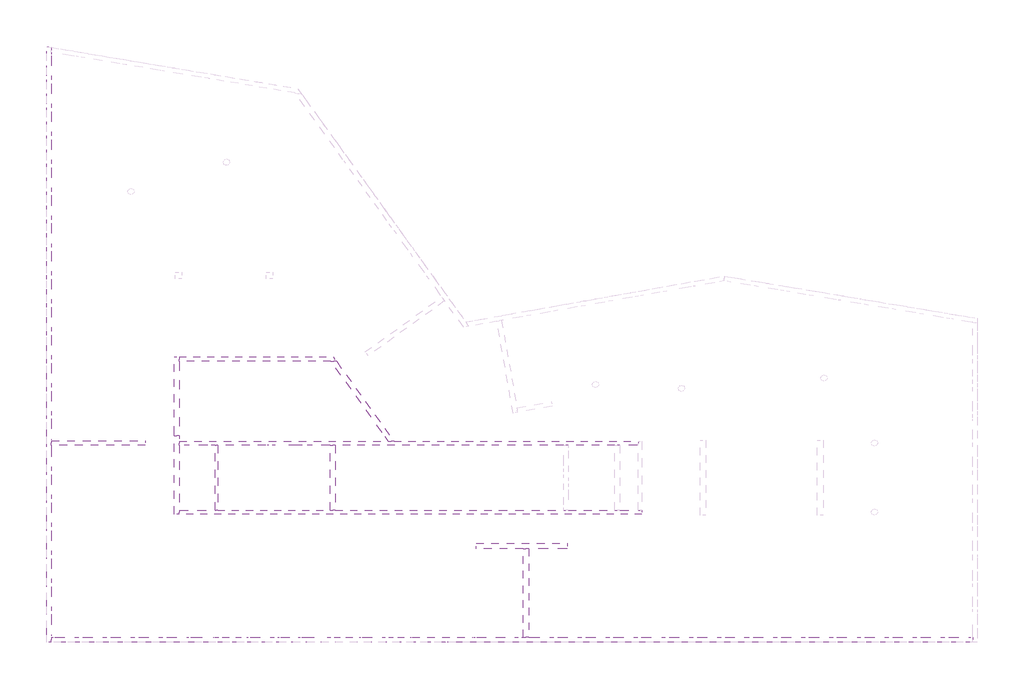
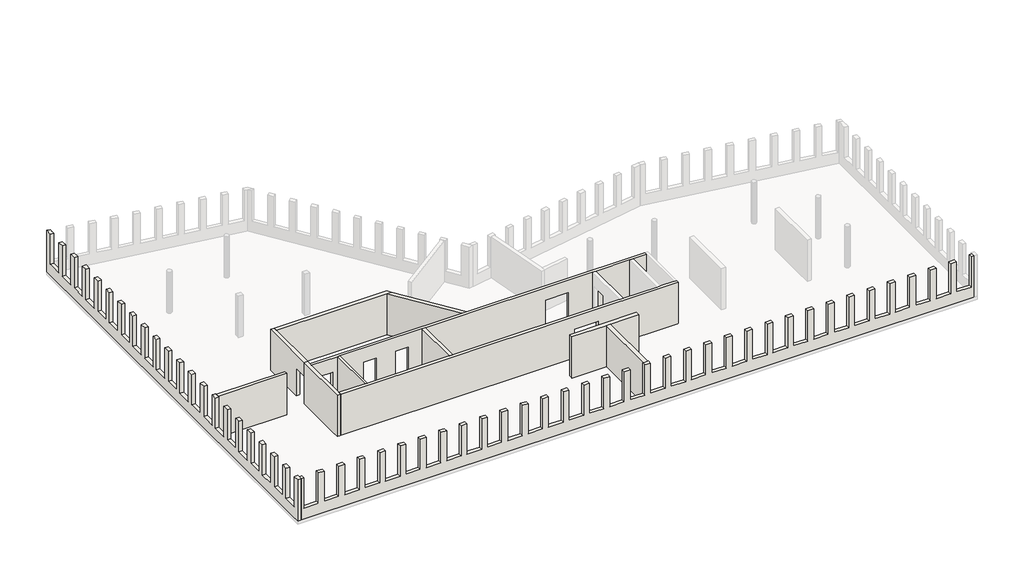
# One storey, part 1 of 2: 13 walls.
"""IFC4 building model written with IfcOpenShell, lengths in millimetres."""

from ifc_helpers import new_model, si_unit, frame, origin, place, context, project, spatial, polyline, outline, extrude, faceted_brep, element, save

model = new_model("IFC4")

# Units and contexts
model_context = context("Model", 3, world=origin())
ifc_project = project(units=[si_unit("LENGTHUNIT", "METRE", prefix="MILLI")], contexts=[model_context])

# Site, building, storey
site = spatial("IfcSite", under=ifc_project)
building = spatial("IfcBuilding", under=site)
storey = spatial("IfcBuildingStorey", under=building, Name="00_EG_OKFB_0,00", Elevation=0.0)

# Walls
placement = place(None, origin())
element("IfcWall", 1, ObjectType="5dki Lochfassade 26cm C30/37", at=placement, inside=storey, context=model_context, shape_type="Brep", body=[
    faceted_brep([(130.0010047, -129.999028, 3310.0), (130.0010047, 130.000972, 3310.0), (130.0010047, 10442.0124295, 3310.0), (130.0010047, 10692.0124295, 3310.0), (130.0010047, 31548.6978518, 3310.0), (130.0010047, 31812.2980067, 3310.0), (130.0010047, 31812.2980067, 6520.0), (130.0010047, 31792.3282645, 6520.0), (130.0010047, 31792.3282645, 4170.0), (130.0010047, 31548.6978518, 4170.0), (130.0010047, 31548.6978518, 6520.0), (130.0010047, 31357.0124158, 6520.0), (130.0010047, 31357.0124158, 4170.0), (130.0010047, 30277.0124158, 4170.0), (130.0010047, 30277.0124158, 6520.0), (130.0010047, 29857.0124158, 6520.0), (130.0010047, 29857.0124158, 4170.0), (130.0010047, 28777.0124158, 4170.0), (130.0010047, 28777.0124158, 6520.0), (130.0010047, 28358.4322867, 6520.0), (130.0010047, 28358.4322867, 4170.0), (130.0010047, 27278.4322867, 4170.0), (130.0010047, 27278.4322867, 6520.0), (130.0010047, 26858.4322867, 6520.0), (130.0010047, 26858.4322867, 4170.0), (130.0010047, 25778.4322867, 4170.0), (130.0010047, 25778.4322867, 6520.0), (130.0010047, 25358.4322867, 6520.0), (130.0010047, 25358.4322867, 4170.0), (130.0010047, 24278.4322867, 4170.0), (130.0010047, 24278.4322867, 6520.0), (130.0010047, 23857.0124158, 6520.0), (130.0010047, 23857.0124158, 4170.0), (130.0010047, 22777.0124158, 4170.0), (130.0010047, 22777.0124158, 6520.0), (130.0010047, 22357.0124158, 6520.0), (130.0010047, 22357.0124158, 4170.0), (130.0010047, 21277.0124158, 4170.0), (130.0010047, 21277.0124158, 6520.0), (130.0010047, 20857.0124158, 6520.0), (130.0010047, 20857.0124158, 4170.0), (130.0010047, 19777.0124158, 4170.0), (130.0010047, 19777.0124158, 6520.0), (130.0010047, 19357.0124158, 6520.0), (130.0010047, 19357.0124158, 4170.0), (130.0010047, 18277.0124158, 4170.0), (130.0010047, 18277.0124158, 6520.0), (130.0010047, 17857.0124158, 6520.0), (130.0010047, 17857.0124158, 4170.0), (130.0010047, 16777.0124158, 4170.0), (130.0010047, 16777.0124158, 6520.0), (130.0010047, 16357.0124158, 6520.0), (130.0010047, 16357.0124158, 4170.0), (130.0010047, 15277.0124158, 4170.0), (130.0010047, 15277.0124158, 6520.0), (130.0010047, 14857.0124158, 6520.0), (130.0010047, 14857.0124158, 4170.0), (130.0010047, 13777.0124158, 4170.0), (130.0010047, 13777.0124158, 6520.0), (130.0010047, 13357.0124158, 6520.0), (130.0010047, 13357.0124158, 4170.0), (130.0010047, 12277.0124158, 4170.0), (130.0010047, 12277.0124158, 6520.0), (130.0010047, 11857.0124158, 6520.0), (130.0010047, 11857.0124158, 4170.0), (130.0010047, 10777.0124158, 4170.0), (130.0010047, 10777.0124158, 6520.0), (130.0010047, 10692.0124295, 6520.0), (130.0010047, 10442.0124295, 6520.0), (130.0010047, 10357.0124158, 6520.0), (130.0010047, 10357.0124158, 4170.0), (130.0010047, 9277.0124158, 4170.0), (130.0010047, 9277.0124158, 6520.0), (130.0010047, 8857.0124158, 6520.0), (130.0010047, 8857.0124158, 4170.0), (130.0010047, 7777.0124158, 4170.0), (130.0010047, 7777.0124158, 6520.0), (130.0010047, 7357.0124158, 6520.0), (130.0010047, 7357.0124158, 4170.0), (130.0010047, 6277.0124158, 4170.0), (130.0010047, 6277.0124158, 6520.0), (130.0010047, 5857.0124158, 6520.0), (130.0010047, 5857.0124158, 4170.0), (130.0010047, 4777.0124158, 4170.0), (130.0010047, 4777.0124158, 6520.0), (130.0010047, 4357.0124158, 6520.0), (130.0010047, 4357.0124158, 4170.0), (130.0010047, 3277.0124158, 4170.0), (130.0010047, 3277.0124158, 6520.0), (130.0010047, 2857.0124158, 6520.0), (130.0010047, 2857.0124158, 4170.0), (130.0010047, 1777.0124158, 4170.0), (130.0010047, 1777.0124158, 6520.0), (130.0010047, 1357.0124158, 6520.0), (130.0010047, 1357.0124158, 4170.0), (130.0010047, 277.0124158, 4170.0), (130.0010047, 277.0124158, 6520.0), (130.0010047, 130.000972, 6520.0), (130.0010047, -129.999028, 6520.0), (-129.9989953, 31855.7150729, 3310.0), (-129.9989953, -129.9990284, 3310.0), (-129.9989953, -129.9990284, 6520.0), (-129.9989953, 277.0124158, 6520.0), (-129.9989953, 277.0124158, 4170.0), (-129.9989953, 1357.0124158, 4170.0), (-129.9989953, 1357.0124158, 6520.0), (-129.9989953, 1777.0124158, 6520.0), (-129.9989953, 1777.0124158, 4170.0), (-129.9989953, 2857.0124158, 4170.0), (-129.9989953, 2857.0124158, 6520.0), (-129.9989953, 3277.0124158, 6520.0), (-129.9989953, 3277.0124158, 4170.0), (-129.9989953, 4357.0124158, 4170.0), (-129.9989953, 4357.0124158, 6520.0), (-129.9989953, 4777.0124158, 6520.0), (-129.9989953, 4777.0124158, 4170.0), (-129.9989953, 5857.0124158, 4170.0), (-129.9989953, 5857.0124158, 6520.0), (-129.9989953, 6277.0124158, 6520.0), (-129.9989953, 6277.0124158, 4170.0), (-129.9989953, 7357.0124158, 4170.0), (-129.9989953, 7357.0124158, 6520.0), (-129.9989953, 7777.0124158, 6520.0), (-129.9989953, 7777.0124158, 4170.0), (-129.9989953, 8857.0124158, 4170.0), (-129.9989953, 8857.0124158, 6520.0), (-129.9989953, 9277.0124158, 6520.0), (-129.9989953, 9277.0124158, 4170.0), (-129.9989953, 10357.0124158, 4170.0), (-129.9989953, 10357.0124158, 6520.0), (-129.9989953, 10777.0124158, 6520.0), (-129.9989953, 10777.0124158, 4170.0), (-129.9989953, 11857.0124158, 4170.0), (-129.9989953, 11857.0124158, 6520.0), (-129.9989953, 12277.0124158, 6520.0), (-129.9989953, 12277.0124158, 4170.0), (-129.9989953, 13357.0124158, 4170.0), (-129.9989953, 13357.0124158, 6520.0), (-129.9989953, 13777.0124158, 6520.0), (-129.9989953, 13777.0124158, 4170.0), (-129.9989953, 14857.0124158, 4170.0), (-129.9989953, 14857.0124158, 6520.0), (-129.9989953, 15277.0124158, 6520.0), (-129.9989953, 15277.0124158, 4170.0), (-129.9989953, 16357.0124158, 4170.0), (-129.9989953, 16357.0124158, 6520.0), (-129.9989953, 16777.0124158, 6520.0), (-129.9989953, 16777.0124158, 4170.0), (-129.9989953, 17857.0124158, 4170.0), (-129.9989953, 17857.0124158, 6520.0), (-129.9989953, 18277.0124158, 6520.0), (-129.9989953, 18277.0124158, 4170.0), (-129.9989953, 19357.0124158, 4170.0), (-129.9989953, 19357.0124158, 6520.0), (-129.9989953, 19777.0124158, 6520.0), (-129.9989953, 19777.0124158, 4170.0), (-129.9989953, 20857.0124158, 4170.0), (-129.9989953, 20857.0124158, 6520.0), (-129.9989953, 21277.0124158, 6520.0), (-129.9989953, 21277.0124158, 4170.0), (-129.9989953, 22357.0124158, 4170.0), (-129.9989953, 22357.0124158, 6520.0), (-129.9989953, 22777.0124158, 6520.0), (-129.9989953, 22777.0124158, 4170.0), (-129.9989953, 23857.0124158, 4170.0), (-129.9989953, 23857.0124158, 6520.0), (-129.9989953, 24278.4322867, 6520.0), (-129.9989953, 24278.4322867, 4170.0), (-129.9989953, 25358.4322867, 4170.0), (-129.9989953, 25358.4322867, 6520.0), (-129.9989953, 25778.4322867, 6520.0), (-129.9989953, 25778.4322867, 4170.0), (-129.9989953, 26858.4322867, 4170.0), (-129.9989953, 26858.4322867, 6520.0), (-129.9989953, 27278.4322867, 6520.0), (-129.9989953, 27278.4322867, 4170.0), (-129.9989953, 28358.4322867, 4170.0), (-129.9989953, 28358.4322867, 6520.0), (-129.9989953, 28777.0124158, 6520.0), (-129.9989953, 28777.0124158, 4170.0), (-129.9989953, 29857.0124158, 4170.0), (-129.9989953, 29857.0124158, 6520.0), (-129.9989953, 30277.0124158, 6520.0), (-129.9989953, 30277.0124158, 4170.0), (-129.9989953, 31357.0124158, 4170.0), (-129.9989953, 31357.0124158, 6520.0), (-129.9989953, 31855.7150729, 6520.0), (90.4211678, 31555.307238, 6520.0), (90.4211678, 31555.307238, 4170.0)], [[[0, 1, 2, 3, 4, 5, 6, 7, 8, 9, 10, 11, 12, 13, 14, 15, 16, 17, 18, 19, 20, 21, 22, 23, 24, 25, 26, 27, 28, 29, 30, 31, 32, 33, 34, 35, 36, 37, 38, 39, 40, 41, 42, 43, 44, 45, 46, 47, 48, 49, 50, 51, 52, 53, 54, 55, 56, 57, 58, 59, 60, 61, 62, 63, 64, 65, 66, 67, 68, 69, 70, 71, 72, 73, 74, 75, 76, 77, 78, 79, 80, 81, 82, 83, 84, 85, 86, 87, 88, 89, 90, 91, 92, 93, 94, 95, 96, 97, 98]], [[99, 100, 101, 102, 103, 104, 105, 106, 107, 108, 109, 110, 111, 112, 113, 114, 115, 116, 117, 118, 119, 120, 121, 122, 123, 124, 125, 126, 127, 128, 129, 130, 131, 132, 133, 134, 135, 136, 137, 138, 139, 140, 141, 142, 143, 144, 145, 146, 147, 148, 149, 150, 151, 152, 153, 154, 155, 156, 157, 158, 159, 160, 161, 162, 163, 164, 165, 166, 167, 168, 169, 170, 171, 172, 173, 174, 175, 176, 177, 178, 179, 180, 181, 182, 183, 184, 185, 186]], [[5, 4, 3, 2, 1, 0, 100, 99]], [[6, 186, 185, 11, 10, 187, 7]], [[101, 98, 97, 96, 102]], [[105, 93, 92, 106]], [[109, 89, 88, 110]], [[113, 85, 84, 114]], [[117, 81, 80, 118]], [[121, 77, 76, 122]], [[125, 73, 72, 126]], [[129, 69, 68, 67, 66, 130]], [[133, 63, 62, 134]], [[137, 59, 58, 138]], [[141, 55, 54, 142]], [[145, 51, 50, 146]], [[149, 47, 46, 150]], [[153, 43, 42, 154]], [[157, 39, 38, 158]], [[161, 35, 34, 162]], [[165, 31, 30, 166]], [[14, 182, 181, 15]], [[18, 178, 177, 19]], [[22, 174, 173, 23]], [[26, 170, 169, 27]], [[6, 5, 99, 186]], [[0, 98, 101, 100]], [[104, 94, 93, 105]], [[95, 103, 102, 96]], [[94, 104, 103, 95]], [[109, 108, 90, 89]], [[107, 106, 92, 91]], [[108, 107, 91, 90]], [[113, 112, 86, 85]], [[111, 110, 88, 87]], [[112, 111, 87, 86]], [[117, 116, 82, 81]], [[115, 114, 84, 83]], [[116, 115, 83, 82]], [[121, 120, 78, 77]], [[119, 118, 80, 79]], [[120, 119, 79, 78]], [[125, 124, 74, 73]], [[123, 122, 76, 75]], [[124, 123, 75, 74]], [[129, 128, 70, 69]], [[127, 126, 72, 71]], [[128, 127, 71, 70]], [[133, 132, 64, 63]], [[131, 130, 66, 65]], [[132, 131, 65, 64]], [[137, 136, 60, 59]], [[135, 134, 62, 61]], [[136, 135, 61, 60]], [[141, 140, 56, 55]], [[139, 138, 58, 57]], [[140, 139, 57, 56]], [[145, 144, 52, 51]], [[143, 142, 54, 53]], [[144, 143, 53, 52]], [[149, 148, 48, 47]], [[147, 146, 50, 49]], [[148, 147, 49, 48]], [[153, 152, 44, 43]], [[151, 150, 46, 45]], [[152, 151, 45, 44]], [[157, 156, 40, 39]], [[155, 154, 42, 41]], [[156, 155, 41, 40]], [[161, 160, 36, 35]], [[159, 158, 38, 37]], [[160, 159, 37, 36]], [[165, 164, 32, 31]], [[163, 162, 34, 33]], [[164, 163, 33, 32]], [[185, 184, 12, 11]], [[183, 182, 14, 13]], [[184, 183, 13, 12]], [[181, 180, 16, 15]], [[179, 178, 18, 17]], [[180, 179, 17, 16]], [[177, 176, 20, 19]], [[175, 174, 22, 21]], [[176, 175, 21, 20]], [[173, 172, 24, 23]], [[171, 170, 26, 25]], [[172, 171, 25, 24]], [[169, 168, 28, 27]], [[167, 166, 30, 29]], [[168, 167, 29, 28]], [[188, 187, 10, 9]], [[187, 188, 8, 7]], [[188, 9, 8]]]),
])
element("IfcWall", 2, ObjectType="5dki Lochfassade 26cm C30/37", at=placement, inside=storey, context=model_context, shape_type="Brep", body=[
    faceted_brep([(49396.9999991, 130.0010483, 4170.0), (49396.9999991, 130.0010483, 6520.0), (49603.9991101, 130.0010486, 6520.0), (49603.9991101, 130.0010486, 3310.0), (25766.9999915, 130.0010117, 3310.0), (25466.9999915, 130.0010113, 3310.0), (130.0010047, 130.000972, 3310.0), (130.0010047, 130.000972, 6520.0), (317.0000012, 130.0009723, 6520.0), (316.999997, 130.0009723, 4170.0), (1397.0000012, 130.000974, 4170.0), (1397.0000069, 130.000974, 6520.0), (1816.9999991, 130.0009747, 6520.0), (1817.0000028, 130.0009747, 4170.0), (2896.9999991, 130.0009763, 4170.0), (2897.0000017, 130.0009763, 6520.0), (3316.9999991, 130.000977, 6520.0), (3316.9999977, 130.000977, 4170.0), (4396.9999991, 130.0009787, 4170.0), (4396.9999966, 130.0009787, 6520.0), (4816.9999991, 130.0009793, 6520.0), (4816.9999991, 130.0009793, 4170.0), (5896.9999991, 130.000981, 4170.0), (5896.9999991, 130.000981, 6520.0), (6316.9999991, 130.0009816, 6520.0), (6316.9999991, 130.0009816, 4170.0), (7396.9999991, 130.0009833, 4170.0), (7396.9999991, 130.0009833, 6520.0), (7816.9999991, 130.0009839, 6520.0), (7816.9999991, 130.0009839, 4170.0), (8896.9999991, 130.0009856, 4170.0), (8896.9999991, 130.0009856, 6520.0), (9316.9999991, 130.0009863, 6520.0), (9316.9999991, 130.0009863, 4170.0), (10396.9999991, 130.0009879, 4170.0), (10396.9999991, 130.0009879, 6520.0), (10816.9999991, 130.0009886, 6520.0), (10816.9999991, 130.0009886, 4170.0), (11896.9999991, 130.0009903, 4170.0), (11896.9999991, 130.0009903, 6520.0), (12316.9999991, 130.0009909, 6520.0), (12316.9999991, 130.0009909, 4170.0), (13396.9999991, 130.0009926, 4170.0), (13396.9999991, 130.0009926, 6520.0), (13816.9999991, 130.0009932, 6520.0), (13816.9999991, 130.0009932, 4170.0), (14896.9999991, 130.0009949, 4170.0), (14896.9999991, 130.0009949, 6520.0), (15316.9999991, 130.0009956, 6520.0), (15316.9999991, 130.0009956, 4170.0), (16396.9999991, 130.0009972, 4170.0), (16396.9999991, 130.0009972, 6520.0), (16816.9999991, 130.0009979, 6520.0), (16816.9999991, 130.0009979, 4170.0), (17896.9999991, 130.0009996, 4170.0), (17896.9999991, 130.0009996, 6520.0), (18316.9999991, 130.0010002, 6520.0), (18316.9999991, 130.0010002, 4170.0), (19396.9999991, 130.0010019, 4170.0), (19396.9999991, 130.0010019, 6520.0), (19816.9999991, 130.0010025, 6520.0), (19816.9999991, 130.0010025, 4170.0), (20896.9999991, 130.0010042, 4170.0), (20896.9999991, 130.0010042, 6520.0), (21316.9999991, 130.0010048, 6520.0), (21316.9999991, 130.0010048, 4170.0), (22396.9999991, 130.0010065, 4170.0), (22396.9999991, 130.0010065, 6520.0), (22816.9999991, 130.0010072, 6520.0), (22816.9999991, 130.0010072, 4170.0), (23896.9999991, 130.0010088, 4170.0), (23896.9999991, 130.0010088, 6520.0), (24316.9999991, 130.0010095, 6520.0), (24316.9999991, 130.0010095, 4170.0), (25396.9999991, 130.0010112, 4170.0), (25396.9999991, 130.0010112, 6520.0), (25466.9999915, 130.0010113, 6520.0), (25766.9999915, 130.0010117, 6520.0), (25816.9999991, 130.0010118, 6520.0), (25816.9999991, 130.0010118, 4170.0), (26896.9999991, 130.0010135, 4170.0), (26896.9999991, 130.0010135, 6520.0), (27316.9999991, 130.0010141, 6520.0), (27316.9999991, 130.0010141, 4170.0), (28396.9999991, 130.0010158, 4170.0), (28396.9999991, 130.0010158, 6520.0), (28816.9999991, 130.0010165, 6520.0), (28816.9999991, 130.0010165, 4170.0), (29896.9999991, 130.0010181, 4170.0), (29896.9999991, 130.0010181, 6520.0), (30316.9999991, 130.0010188, 6520.0), (30316.9999991, 130.0010188, 4170.0), (31396.9999991, 130.0010205, 4170.0), (31396.9999991, 130.0010205, 6520.0), (31816.9999991, 130.0010211, 6520.0), (31816.9999991, 130.0010211, 4170.0), (32896.9999991, 130.0010228, 4170.0), (32896.9999991, 130.0010228, 6520.0), (33316.9999991, 130.0010234, 6520.0), (33316.9999991, 130.0010234, 4170.0), (34396.9999991, 130.0010251, 4170.0), (34396.9999991, 130.0010251, 6520.0), (34816.9999991, 130.0010258, 6520.0), (34816.9999991, 130.0010258, 4170.0), (35896.9999991, 130.0010274, 4170.0), (35896.9999991, 130.0010274, 6520.0), (36316.9999991, 130.0010281, 6520.0), (36316.9999991, 130.0010281, 4170.0), (37396.9999991, 130.0010297, 4170.0), (37396.9999991, 130.0010297, 6520.0), (37816.9999991, 130.0010304, 6520.0), (37816.9999991, 130.0010304, 4170.0), (38896.9999991, 130.0010321, 4170.0), (38896.9999991, 130.0010321, 6520.0), (39316.9999991, 130.0010327, 6520.0), (39316.9999991, 130.0010327, 4170.0), (40396.9999991, 130.0010344, 4170.0), (40396.9999991, 130.0010344, 6520.0), (40816.9999991, 130.001035, 6520.0), (40816.9999991, 130.001035, 4170.0), (41896.9999991, 130.0010367, 4170.0), (41896.9999991, 130.0010367, 6520.0), (42316.9999991, 130.0010374, 6520.0), (42316.9999991, 130.0010374, 4170.0), (43396.9999991, 130.001039, 4170.0), (43396.9999991, 130.001039, 6520.0), (43816.9999991, 130.0010397, 6520.0), (43816.9999991, 130.0010397, 4170.0), (44896.9999991, 130.0010414, 4170.0), (44896.9999991, 130.0010414, 6520.0), (45316.9999991, 130.001042, 6520.0), (45316.9999991, 130.001042, 4170.0), (46396.9999991, 130.0010437, 4170.0), (46396.9999991, 130.0010437, 6520.0), (46816.9999991, 130.0010443, 6520.0), (46816.9999991, 130.0010443, 4170.0), (47896.9999991, 130.001046, 4170.0), (47896.9999991, 130.001046, 6520.0), (48316.9999991, 130.0010467, 6520.0), (48316.9999991, 130.0010467, 4170.0), (49603.9991105, -129.9989514, 6520.0), (49396.9999995, -129.9989517, 6520.0), (49396.9999995, -129.9989517, 4170.0), (48316.9999995, -129.9989533, 4170.0), (48316.9999995, -129.9989533, 6520.0), (47896.9999995, -129.998954, 6520.0), (47896.9999995, -129.998954, 4170.0), (46816.9999995, -129.9989557, 4170.0), (46816.9999995, -129.9989557, 6520.0), (46396.9999995, -129.9989563, 6520.0), (46396.9999995, -129.9989563, 4170.0), (45316.9999995, -129.998958, 4170.0), (45316.9999995, -129.998958, 6520.0), (44896.9999995, -129.9989586, 6520.0), (44896.9999995, -129.9989586, 4170.0), (43816.9999995, -129.9989603, 4170.0), (43816.9999995, -129.9989603, 6520.0), (43396.9999995, -129.998961, 6520.0), (43396.9999995, -129.998961, 4170.0), (42316.9999995, -129.9989626, 4170.0), (42316.9999995, -129.9989626, 6520.0), (41896.9999995, -129.9989633, 6520.0), (41896.9999995, -129.9989633, 4170.0), (40816.9999995, -129.998965, 4170.0), (40816.9999995, -129.998965, 6520.0), (40396.9999995, -129.9989656, 6520.0), (40396.9999995, -129.9989656, 4170.0), (39316.9999995, -129.9989673, 4170.0), (39316.9999995, -129.9989673, 6520.0), (38896.9999995, -129.9989679, 6520.0), (38896.9999995, -129.9989679, 4170.0), (37816.9999995, -129.9989696, 4170.0), (37816.9999995, -129.9989696, 6520.0), (37396.9999995, -129.9989703, 6520.0), (37396.9999995, -129.9989703, 4170.0), (36316.9999995, -129.9989719, 4170.0), (36316.9999995, -129.9989719, 6520.0), (35896.9999995, -129.9989726, 6520.0), (35896.9999995, -129.9989726, 4170.0), (34816.9999995, -129.9989742, 4170.0), (34816.9999995, -129.9989742, 6520.0), (34396.9999995, -129.9989749, 6520.0), (34396.9999995, -129.9989749, 4170.0), (33316.9999995, -129.9989766, 4170.0), (33316.9999995, -129.9989766, 6520.0), (32896.9999995, -129.9989772, 6520.0), (32896.9999995, -129.9989772, 4170.0), (31816.9999995, -129.9989789, 4170.0), (31816.9999995, -129.9989789, 6520.0), (31396.9999995, -129.9989795, 6520.0), (31396.9999995, -129.9989795, 4170.0), (30316.9999995, -129.9989812, 4170.0), (30316.9999995, -129.9989812, 6520.0), (29896.9999995, -129.9989819, 6520.0), (29896.9999995, -129.9989819, 4170.0), (28816.9999995, -129.9989835, 4170.0), (28816.9999995, -129.9989835, 6520.0), (28396.9999995, -129.9989842, 6520.0), (28396.9999995, -129.9989842, 4170.0), (27316.9999995, -129.9989859, 4170.0), (27316.9999995, -129.9989859, 6520.0), (26896.9999995, -129.9989865, 6520.0), (26896.9999995, -129.9989865, 4170.0), (25816.9999995, -129.9989882, 4170.0), (25816.9999995, -129.9989882, 6520.0), (25396.9999995, -129.9989888, 6520.0), (25396.9999995, -129.9989888, 4170.0), (24316.9999995, -129.9989905, 4170.0), (24316.9999995, -129.9989905, 6520.0), (23896.9999995, -129.9989912, 6520.0), (23896.9999995, -129.9989912, 4170.0), (22816.9999995, -129.9989928, 4170.0), (22816.9999995, -129.9989928, 6520.0), (22396.9999995, -129.9989935, 6520.0), (22396.9999995, -129.9989935, 4170.0), (21316.9999995, -129.9989952, 4170.0), (21316.9999995, -129.9989952, 6520.0), (20896.9999995, -129.9989958, 6520.0), (20896.9999995, -129.9989958, 4170.0), (19816.9999995, -129.9989975, 4170.0), (19816.9999995, -129.9989975, 6520.0), (19396.9999995, -129.9989981, 6520.0), (19396.9999995, -129.9989981, 4170.0), (18316.9999995, -129.9989998, 4170.0), (18316.9999995, -129.9989998, 6520.0), (17896.9999995, -129.9990004, 6520.0), (17896.9999995, -129.9990004, 4170.0), (16816.9999995, -129.9990021, 4170.0), (16816.9999995, -129.9990021, 6520.0), (16396.9999995, -129.9990028, 6520.0), (16396.9999995, -129.9990028, 4170.0), (15316.9999995, -129.9990044, 4170.0), (15316.9999995, -129.9990044, 6520.0), (14896.9999995, -129.9990051, 6520.0), (14896.9999995, -129.9990051, 4170.0), (13816.9999995, -129.9990068, 4170.0), (13816.9999995, -129.9990068, 6520.0), (13396.9999995, -129.9990074, 6520.0), (13396.9999995, -129.9990074, 4170.0), (12316.9999995, -129.9990091, 4170.0), (12316.9999995, -129.9990091, 6520.0), (11896.9999995, -129.9990097, 6520.0), (11896.9999995, -129.9990097, 4170.0), (10816.9999995, -129.9990114, 4170.0), (10816.9999995, -129.9990114, 6520.0), (10396.9999995, -129.9990121, 6520.0), (10396.9999995, -129.9990121, 4170.0), (9316.9999995, -129.9990137, 4170.0), (9316.9999995, -129.9990137, 6520.0), (8896.9999995, -129.9990144, 6520.0), (8896.9999995, -129.9990144, 4170.0), (7816.9999995, -129.9990161, 4170.0), (7816.9999995, -129.9990161, 6520.0), (7396.9999995, -129.9990167, 6520.0), (7396.9999995, -129.9990167, 4170.0), (6316.9999995, -129.9990184, 4170.0), (6316.9999995, -129.9990184, 6520.0), (5896.9999995, -129.999019, 6520.0), (5896.9999995, -129.999019, 4170.0), (4816.9999995, -129.9990207, 4170.0), (4816.9999995, -129.9990207, 6520.0), (4396.9999995, -129.9990213, 6520.0), (4396.9999966, -129.9990213, 4170.0), (3316.9999995, -129.999023, 4170.0), (3316.9999977, -129.999023, 6520.0), (2896.9999995, -129.9990237, 6520.0), (2897.0000017, -129.9990237, 4170.0), (1816.9999995, -129.9990253, 4170.0), (1817.0000028, -129.9990253, 6520.0), (1397.0000016, -129.999026, 6520.0), (1397.0000069, -129.999026, 4170.0), (317.0000016, -129.9990277, 4170.0), (316.999997, -129.9990277, 6520.0), (130.0010047, -129.999028, 6520.0), (130.0010047, -129.999028, 3310.0), (49603.9991105, -129.9989514, 3310.0)], [[[0, 1, 2, 3, 4, 5, 6, 7, 8, 9, 10, 11, 12, 13, 14, 15, 16, 17, 18, 19, 20, 21, 22, 23, 24, 25, 26, 27, 28, 29, 30, 31, 32, 33, 34, 35, 36, 37, 38, 39, 40, 41, 42, 43, 44, 45, 46, 47, 48, 49, 50, 51, 52, 53, 54, 55, 56, 57, 58, 59, 60, 61, 62, 63, 64, 65, 66, 67, 68, 69, 70, 71, 72, 73, 74, 75, 76, 77, 78, 79, 80, 81, 82, 83, 84, 85, 86, 87, 88, 89, 90, 91, 92, 93, 94, 95, 96, 97, 98, 99, 100, 101, 102, 103, 104, 105, 106, 107, 108, 109, 110, 111, 112, 113, 114, 115, 116, 117, 118, 119, 120, 121, 122, 123, 124, 125, 126, 127, 128, 129, 130, 131, 132, 133, 134, 135, 136, 137, 138, 139]], [[140, 141, 142, 143, 144, 145, 146, 147, 148, 149, 150, 151, 152, 153, 154, 155, 156, 157, 158, 159, 160, 161, 162, 163, 164, 165, 166, 167, 168, 169, 170, 171, 172, 173, 174, 175, 176, 177, 178, 179, 180, 181, 182, 183, 184, 185, 186, 187, 188, 189, 190, 191, 192, 193, 194, 195, 196, 197, 198, 199, 200, 201, 202, 203, 204, 205, 206, 207, 208, 209, 210, 211, 212, 213, 214, 215, 216, 217, 218, 219, 220, 221, 222, 223, 224, 225, 226, 227, 228, 229, 230, 231, 232, 233, 234, 235, 236, 237, 238, 239, 240, 241, 242, 243, 244, 245, 246, 247, 248, 249, 250, 251, 252, 253, 254, 255, 256, 257, 258, 259, 260, 261, 262, 263, 264, 265, 266, 267, 268, 269, 270, 271, 272, 273, 274, 275]], [[6, 5, 4, 3, 275, 274]], [[7, 273, 272, 8]], [[15, 265, 264, 16]], [[268, 12, 11, 269]], [[261, 260, 20, 19]], [[257, 256, 24, 23]], [[253, 252, 28, 27]], [[249, 248, 32, 31]], [[245, 244, 36, 35]], [[241, 240, 40, 39]], [[237, 236, 44, 43]], [[233, 232, 48, 47]], [[229, 228, 52, 51]], [[225, 224, 56, 55]], [[221, 220, 60, 59]], [[217, 216, 64, 63]], [[213, 212, 68, 67]], [[209, 208, 72, 71]], [[205, 204, 78, 77, 76, 75]], [[201, 200, 82, 81]], [[197, 196, 86, 85]], [[193, 192, 90, 89]], [[189, 188, 94, 93]], [[185, 184, 98, 97]], [[181, 180, 102, 101]], [[177, 176, 106, 105]], [[173, 172, 110, 109]], [[169, 168, 114, 113]], [[165, 164, 118, 117]], [[161, 160, 122, 121]], [[157, 156, 126, 125]], [[153, 152, 130, 129]], [[149, 148, 134, 133]], [[138, 137, 145, 144]], [[2, 1, 141, 140]], [[7, 6, 274, 273]], [[3, 2, 140, 275]], [[10, 270, 269, 11]], [[271, 9, 8, 272]], [[270, 10, 9, 271]], [[14, 266, 265, 15]], [[267, 13, 12, 268]], [[266, 14, 13, 267]], [[18, 262, 261, 19]], [[263, 17, 16, 264]], [[262, 18, 17, 263]], [[23, 22, 258, 257]], [[21, 20, 260, 259]], [[22, 21, 259, 258]], [[27, 26, 254, 253]], [[25, 24, 256, 255]], [[26, 25, 255, 254]], [[31, 30, 250, 249]], [[29, 28, 252, 251]], [[30, 29, 251, 250]], [[35, 34, 246, 245]], [[33, 32, 248, 247]], [[34, 33, 247, 246]], [[39, 38, 242, 241]], [[37, 36, 244, 243]], [[38, 37, 243, 242]], [[43, 42, 238, 237]], [[41, 40, 240, 239]], [[42, 41, 239, 238]], [[47, 46, 234, 233]], [[45, 44, 236, 235]], [[46, 45, 235, 234]], [[51, 50, 230, 229]], [[49, 48, 232, 231]], [[50, 49, 231, 230]], [[55, 54, 226, 225]], [[53, 52, 228, 227]], [[54, 53, 227, 226]], [[59, 58, 222, 221]], [[57, 56, 224, 223]], [[58, 57, 223, 222]], [[63, 62, 218, 217]], [[61, 60, 220, 219]], [[62, 61, 219, 218]], [[67, 66, 214, 213]], [[65, 64, 216, 215]], [[66, 65, 215, 214]], [[71, 70, 210, 209]], [[69, 68, 212, 211]], [[70, 69, 211, 210]], [[75, 74, 206, 205]], [[73, 72, 208, 207]], [[74, 73, 207, 206]], [[81, 80, 202, 201]], [[79, 78, 204, 203]], [[80, 79, 203, 202]], [[85, 84, 198, 197]], [[83, 82, 200, 199]], [[84, 83, 199, 198]], [[89, 88, 194, 193]], [[87, 86, 196, 195]], [[88, 87, 195, 194]], [[93, 92, 190, 189]], [[91, 90, 192, 191]], [[92, 91, 191, 190]], [[97, 96, 186, 185]], [[95, 94, 188, 187]], [[96, 95, 187, 186]], [[101, 100, 182, 181]], [[99, 98, 184, 183]], [[100, 99, 183, 182]], [[105, 104, 178, 177]], [[103, 102, 180, 179]], [[104, 103, 179, 178]], [[109, 108, 174, 173]], [[107, 106, 176, 175]], [[108, 107, 175, 174]], [[113, 112, 170, 169]], [[111, 110, 172, 171]], [[112, 111, 171, 170]], [[117, 116, 166, 165]], [[115, 114, 168, 167]], [[116, 115, 167, 166]], [[121, 120, 162, 161]], [[119, 118, 164, 163]], [[120, 119, 163, 162]], [[125, 124, 158, 157]], [[123, 122, 160, 159]], [[124, 123, 159, 158]], [[129, 128, 154, 153]], [[127, 126, 156, 155]], [[128, 127, 155, 154]], [[133, 132, 150, 149]], [[131, 130, 152, 151]], [[132, 131, 151, 150]], [[137, 136, 146, 145]], [[135, 134, 148, 147]], [[136, 135, 147, 146]], [[144, 143, 139, 138]], [[142, 141, 1, 0]], [[143, 142, 0, 139]]]),
])
element("IfcWall", 3, ObjectType="5dki STB-Wand Kern 25cm C30/37", at=placement, inside=storey, context=model_context, shape_type="Brep", body=[
    faceted_brep([(6989.9999766, 15192.0124447, 6520.0), (6989.9999766, 14942.0124447, 6520.0), (6989.9999766, 10947.0136187, 6520.0), (6989.9999766, 10947.0136187, 5445.0), (6989.9999766, 11957.013616, 5445.0), (6989.9999766, 11957.013616, 3310.0), (6989.9999766, 14942.0124447, 3310.0), (6989.9999766, 15192.0124447, 3310.0), (6739.9999766, 10947.0136187, 6520.0), (6739.9999766, 15192.0124447, 6520.0), (6739.9999766, 15192.0124447, 3310.0), (6739.9999766, 11957.013616, 3310.0), (6739.9999766, 11957.013616, 5445.0), (6739.9999766, 10947.0136187, 5445.0)], [[[0, 1, 2, 3, 4, 5, 6, 7]], [[8, 9, 10, 11, 12, 13]], [[10, 7, 6, 5, 11]], [[2, 1, 0, 9, 8]], [[2, 8, 13, 3]], [[0, 7, 10, 9]], [[4, 12, 11, 5]], [[12, 4, 3, 13]]]),
])
element("IfcWall", 4, ObjectType="5dki STB-Wand Kern 25cm C30/37", at=placement, inside=storey, context=model_context, shape_type="Brep", body=[
    faceted_brep([(6989.9999766, 14942.0124447, 3310.0), (15141.8279932, 14942.0124447, 3310.0), (15449.8792779, 14942.0124447, 3310.0), (15449.8792779, 14942.0124447, 6520.0), (15141.8279932, 14942.0124447, 6520.0), (6989.9999766, 14942.0124447, 6520.0), (6989.9999766, 15192.0124447, 3310.0), (6989.9999766, 15192.0124447, 6520.0), (15269.8915173, 15192.0124447, 6520.0), (15269.8915173, 15192.0124447, 3310.0)], [[[0, 1, 2, 3, 4, 5]], [[6, 7, 8, 9]], [[2, 1, 0, 6, 9]], [[5, 4, 3, 8, 7]], [[0, 5, 7, 6]], [[3, 2, 9, 8]]]),
])
element("IfcWall", 5, ObjectType="5dki STB-Wand Kern 25cm C30/37", at=placement, inside=storey, context=model_context, shape_type="Brep", body=[
    faceted_brep([(18223.2182524, 10662.0127257, 6520.0), (15141.8279932, 14942.0124447, 6520.0), (15141.8279932, 14942.0124447, 3310.0), (17305.3310134, 11936.9428041, 3310.0), (17305.3310134, 11936.9428041, 5445.0), (17895.4523577, 11117.2740911, 5445.0), (17895.4523577, 11117.2740911, 3310.0), (18223.2182524, 10662.0127257, 3310.0), (15449.8792779, 14942.0124447, 6520.0), (18531.2695366, 10662.0127262, 6520.0), (18531.2695366, 10662.0127262, 3310.0), (18098.340653, 11263.3437308, 3310.0), (18098.340653, 11263.3437308, 5445.0), (17508.2193087, 12083.0124438, 5445.0), (17508.2193087, 12083.0124438, 3310.0), (15449.8792779, 14942.0124447, 3310.0)], [[[0, 1, 2, 3, 4, 5, 6, 7]], [[8, 9, 10, 11, 12, 13, 14, 15]], [[2, 15, 14, 3]], [[10, 7, 6, 11]], [[1, 0, 9, 8]], [[2, 1, 8, 15]], [[0, 7, 10, 9]], [[13, 4, 3, 14]], [[4, 13, 12, 5]], [[5, 12, 11, 6]]]),
])
element("IfcWall", 6, ObjectType="5dki STB-Wand Kern 25cm C30/37", at=placement, inside=storey, context=model_context, shape_type="Brep", body=[
    faceted_brep([(6739.9995723, 10947.0136187, 3310.0), (6739.9995723, 6740.0000204, 3310.0), (6739.9995723, 6740.0000204, 6520.0), (6739.9995723, 10947.0136187, 6520.0), (6739.9995723, 10947.0136187, 5445.0), (6989.9995723, 10947.0136187, 3310.0), (6989.9995723, 10947.0136187, 5445.0), (6989.9995723, 10947.0136187, 6520.0), (6989.9995723, 10662.0127052, 6520.0), (6989.9995723, 10442.0127052, 6520.0), (6989.9995723, 6960.0000208, 6520.0), (6989.9995723, 6740.0000208, 6520.0), (6989.9995723, 6740.0000208, 3310.0), (6989.9995723, 6960.0000208, 3310.0), (6989.9995723, 10442.0127052, 3310.0), (6989.9995723, 10662.0127052, 3310.0)], [[[0, 1, 2, 3, 4]], [[5, 6, 7, 8, 9, 10, 11, 12, 13, 14, 15]], [[1, 0, 5, 15, 14, 13, 12]], [[3, 2, 11, 10, 9, 8, 7]], [[0, 4, 3, 7, 6, 5]], [[2, 1, 12, 11]]]),
])
element("IfcWall", 7, ObjectType="5dki STB-Wand Kern 22cm C30/37", at=placement, inside=storey, context=model_context, shape_type="Brep", body=[
    faceted_brep([(31841.999935, 6740.0000516, 6520.0), (6989.9995723, 6740.0000208, 6520.0), (6989.9995723, 6740.0000208, 3310.0), (24166.9999591, 6740.0000421, 3310.0), (24166.999888, 6740.0000421, 5570.0), (25926.9999591, 6740.0000443, 5570.0), (25927.000338, 6740.0000443, 3310.0), (31841.999935, 6740.0000516, 3310.0), (6989.9995723, 6960.0000208, 6520.0), (8916.9999886, 6960.0000232, 6520.0), (9066.9999886, 6960.0000233, 6520.0), (15117.0008797, 6960.0000309, 6520.0), (15367.0008797, 6960.0000312, 6520.0), (27641.9999886, 6960.0000464, 6520.0), (27891.9999886, 6960.0000467, 6520.0), (30391.9999891, 6960.0000498, 6520.0), (30641.9999891, 6960.0000501, 6520.0), (31641.9999382, 6960.0000514, 6520.0), (31841.9999382, 6960.0000516, 6520.0), (31841.9999382, 6960.0000516, 3310.0), (31641.9999382, 6960.0000514, 3310.0), (30641.9999891, 6960.0000501, 3310.0), (30391.9999891, 6960.0000498, 3310.0), (27891.9999886, 6960.0000467, 3310.0), (27641.9999886, 6960.0000464, 3310.0), (25926.9999588, 6960.0000443, 3310.0), (25927.000338, 6960.0000443, 5570.0), (24166.9999588, 6960.0000421, 5570.0), (24166.999888, 6960.0000421, 3310.0), (15367.0008797, 6960.0000312, 3310.0), (15117.0008797, 6960.0000309, 3310.0), (9066.9999886, 6960.0000233, 3310.0), (8916.9999886, 6960.0000232, 3310.0), (6989.9995723, 6960.0000208, 3310.0)], [[[0, 1, 2, 3, 4, 5, 6, 7]], [[8, 9, 10, 11, 12, 13, 14, 15, 16, 17, 18, 19, 20, 21, 22, 23, 24, 25, 26, 27, 28, 29, 30, 31, 32, 33]], [[2, 33, 32, 31, 30, 29, 28, 3]], [[19, 7, 6, 25, 24, 23, 22, 21, 20]], [[1, 0, 18, 17, 16, 15, 14, 13, 12, 11, 10, 9, 8]], [[2, 1, 8, 33]], [[0, 7, 19, 18]], [[5, 26, 25, 6]], [[26, 5, 4, 27]], [[27, 4, 3, 28]]]),
])
element("IfcWall", 8, ObjectType="5dki STB-Wand Kern 22cm C30/37", at=placement, inside=storey, context=model_context, shape_type="Brep", body=[
    faceted_brep([(6989.9995723, 10662.0127052, 6520.0), (18223.2182524, 10662.0127257, 6520.0), (18531.2695366, 10662.0127262, 6520.0), (31641.9999912, 10662.0127502, 6520.0), (31641.9999912, 10662.0127502, 3310.0), (25926.999945, 10662.0127397, 3310.0), (25927.0000254, 10662.0127397, 5570.0), (24166.999945, 10662.0127365, 5570.0), (24166.9998144, 10662.0127365, 3310.0), (18531.2695366, 10662.0127262, 3310.0), (18223.2182524, 10662.0127257, 3310.0), (14152.0004935, 10662.0127182, 3310.0), (14152.0007698, 10662.0127182, 5445.0), (13142.0004935, 10662.0127164, 5445.0), (13142.0009721, 10662.0127164, 3310.0), (11796.9999806, 10662.0127139, 3310.0), (11796.9997327, 10662.0127139, 5445.0), (10786.9999806, 10662.0127121, 5445.0), (10786.999935, 10662.0127121, 3310.0), (8540.0010342, 10662.012708, 3310.0), (8540.000485, 10662.012708, 5445.0), (7530.0010342, 10662.0127061, 5445.0), (7530.0006873, 10662.0127061, 3310.0), (6989.9995723, 10662.0127052, 3310.0), (31641.9999881, 10442.0127502, 6520.0), (30641.9999891, 10442.0127483, 6520.0), (30391.9999891, 10442.0127479, 6520.0), (27891.9999829, 10442.0127433, 6520.0), (27641.9999829, 10442.0127429, 6520.0), (15367.0008797, 10442.0127204, 6520.0), (15117.0008797, 10442.01272, 6520.0), (9066.9999886, 10442.0127089, 6520.0), (8916.9999886, 10442.0127087, 6520.0), (6989.9995723, 10442.0127052, 6520.0), (6989.9995723, 10442.0127052, 3310.0), (7530.0010346, 10442.0127061, 3310.0), (7530.0006873, 10442.0127061, 5445.0), (8540.0010346, 10442.012708, 5445.0), (8540.000485, 10442.012708, 3310.0), (8916.9999886, 10442.0127087, 3310.0), (9066.9999886, 10442.0127089, 3310.0), (10786.999981, 10442.0127121, 3310.0), (10786.999935, 10442.0127121, 5445.0), (11796.999981, 10442.0127139, 5445.0), (11796.9997327, 10442.0127139, 3310.0), (13142.0004939, 10442.0127164, 3310.0), (13142.0009721, 10442.0127164, 5445.0), (14152.0004939, 10442.0127182, 5445.0), (14152.0007698, 10442.0127182, 3310.0), (15117.0008797, 10442.01272, 3310.0), (15367.0008797, 10442.0127204, 3310.0), (24166.9999454, 10442.0127365, 3310.0), (24166.9998144, 10442.0127365, 5570.0), (25926.9999454, 10442.0127397, 5570.0), (25927.0000254, 10442.0127397, 3310.0), (27641.9999829, 10442.0127429, 3310.0), (27891.9999829, 10442.0127433, 3310.0), (30391.9999891, 10442.0127479, 3310.0), (30641.9999891, 10442.0127483, 3310.0), (31641.9999881, 10442.0127502, 3310.0)], [[[0, 1, 2, 3, 4, 5, 6, 7, 8, 9, 10, 11, 12, 13, 14, 15, 16, 17, 18, 19, 20, 21, 22, 23]], [[24, 25, 26, 27, 28, 29, 30, 31, 32, 33, 34, 35, 36, 37, 38, 39, 40, 41, 42, 43, 44, 45, 46, 47, 48, 49, 50, 51, 52, 53, 54, 55, 56, 57, 58, 59]], [[34, 23, 22, 35]], [[4, 59, 58, 57, 56, 55, 54, 5]], [[8, 51, 50, 49, 48, 11, 10, 9]], [[18, 41, 40, 39, 38, 19]], [[44, 15, 14, 45]], [[3, 2, 1, 0, 33, 32, 31, 30, 29, 28, 27, 26, 25, 24]], [[0, 23, 34, 33]], [[4, 3, 24, 59]], [[53, 6, 5, 54]], [[6, 53, 52, 7]], [[7, 52, 51, 8]], [[17, 42, 41, 18]], [[42, 17, 16, 43]], [[43, 16, 15, 44]], [[13, 46, 45, 14]], [[46, 13, 12, 47]], [[47, 12, 11, 48]], [[21, 36, 35, 22]], [[36, 21, 20, 37]], [[37, 20, 19, 38]]]),
])
element("IfcWall", 9, ObjectType="5dki STB-Wand Kern 25cm C30/37", at=placement, inside=storey, context=model_context, shape_type="SweptSolid", body=[
    extrude(outline(polyline([(15117.0008797, 6960.0000309), (15117.0008797, 10442.01272), (15367.0008797, 10442.0127204), (15367.0008797, 6960.0000312), (15117.0008797, 6960.0000309)])), frame((0.0, 0.0, 3310.0), z_axis=(0.0, 0.0, 1.0), x_axis=(1.0, 0.0, 0.0)), (0.0, 0.0, 1.0), 3210.0),
])
element("IfcWall", 10, ObjectType="5dki STB-Wand Kern 15cm C30/37", at=placement, inside=storey, context=model_context, shape_type="SweptSolid", body=[
    extrude(outline(polyline([(8916.9999886, 6960.0000232), (8916.9999886, 10442.0127087), (9066.9999886, 10442.0127089), (9066.9999886, 6960.0000233), (8916.9999886, 6960.0000232)])), frame((0.0, 0.0, 3310.0), z_axis=(0.0, 0.0, 1.0), x_axis=(1.0, 0.0, 0.0)), (0.0, 0.0, 1.0), 3210.0),
])
element("IfcWall", 11, ObjectType="5dki STB-Wand 25cm C30/37", at=placement, inside=storey, context=model_context, shape_type="SweptSolid", body=[
    extrude(outline(polyline([(130.0010047, 10692.0124295), (5179.9999831, 10692.0124295), (5179.9999831, 10442.0124295), (130.0010047, 10442.0124295), (130.0010047, 10692.0124295)])), frame((0.0, 0.0, 3310.0), z_axis=(0.0, 0.0, 1.0), x_axis=(1.0, 0.0, 0.0)), (0.0, 0.0, 1.0), 3210.0),
])
element("IfcWall", 12, ObjectType="5dki STB-Wand 30cm C30/37", at=placement, inside=storey, context=model_context, shape_type="Brep", body=[
    faceted_brep([(22936.4905033, 4880.0000432, 3310.0), (25466.9999915, 4880.0000432, 3310.0), (25766.9999915, 4880.0000432, 3310.0), (27842.0010332, 4880.0000432, 3310.0), (27842.0010332, 4880.0000432, 6520.0), (25766.9999915, 4880.0000432, 6520.0), (25466.9999915, 4880.0000432, 6520.0), (22936.4905033, 4880.0000432, 6520.0), (22936.4905033, 5180.0000432, 3310.0), (22936.4905033, 5180.0000432, 6520.0), (27842.0010332, 5180.0000432, 6520.0), (27842.0010332, 5180.0000432, 3310.0)], [[[0, 1, 2, 3, 4, 5, 6, 7]], [[8, 9, 10, 11]], [[3, 2, 1, 0, 8, 11]], [[4, 3, 11, 10]], [[7, 6, 5, 4, 10, 9]], [[0, 7, 9, 8]]]),
])
element("IfcWall", 13, ObjectType="5dki STB-Wand 30cm C30/37", at=placement, inside=storey, context=model_context, shape_type="SweptSolid", body=[
    extrude(outline(polyline([(25466.9999915, 130.0010113), (25466.9999915, 4880.0000432), (25766.9999915, 4880.0000432), (25766.9999915, 130.0010117), (25466.9999915, 130.0010113)])), frame((0.0, 0.0, 3310.0), z_axis=(0.0, 0.0, 1.0), x_axis=(1.0, 0.0, 0.0)), (0.0, 0.0, 1.0), 3210.0),
])

save(model, "model.ifc")

# Revit data of these elements
# Type "5dki Lochfassade 26cm C30/37"
#   Type Comments = ""
#   Description = ""
#   cpiComponentType = "Wall"
#   cpiFitMatchKey = "5D-KI-STB-OB-W-LF"
#   5d Materialgüte = "C35/45"
#   Filter Tragend / Nichttragend = yes
#   5dki WU = no
#   Layers, outside or top first: 0.260 m "5d Beton - Stahlbeton" (function 1)
# Type "5dki STB-Wand Kern 25cm C30/37"
#   Type Comments = ""
#   Description = ""
#   cpiComponentType = "Wall"
#   cpiFitMatchKey = "5D-KI-STB-OB-W-K"
#   5d Materialgüte = "C30/37"
#   Filter Tragend / Nichttragend = yes
#   5dki WU = no
#   Layers, outside or top first: 0.250 m "5d Beton - Stahlbeton" (function 1)
# Type "5dki STB-Wand Kern 22cm C30/37"
#   Type Comments = ""
#   Description = ""
#   cpiComponentType = "Wall"
#   cpiFitMatchKey = "5D-KI-STB-OB-W-K"
#   5d Materialgüte = "C30/37"
#   Filter Tragend / Nichttragend = yes
#   5dki WU = no
#   Layers, outside or top first: 0.220 m "5d Beton - Stahlbeton" (function 1)
# Type "5dki STB-Wand Kern 15cm C30/37"
#   Type Comments = ""
#   Description = ""
#   cpiComponentType = "Wall"
#   cpiFitMatchKey = "5D-KI-STB-OB-W-K"
#   5d Materialgüte = "C30/37"
#   Filter Tragend / Nichttragend = yes
#   5dki WU = no
#   Layers, outside or top first: 0.150 m "5d Beton - Stahlbeton" (function 1)
# Type "5dki STB-Wand 25cm C30/37"
#   Type Comments = ""
#   Description = ""
#   cpiComponentType = "Wall"
#   cpiFitMatchKey = "5D-KI-STB-OB-W"
#   5d Materialgüte = "C30/37"
#   Filter Tragend / Nichttragend = yes
#   5dki WU = no
#   Layers, outside or top first: 0.250 m "5d Beton - Stahlbeton" (function 1)
# Type "5dki STB-Wand 30cm C30/37"
#   Type Comments = ""
#   Description = ""
#   cpiComponentType = "Wall"
#   cpiFitMatchKey = "5D-KI-STB-OB-W"
#   5d Materialgüte = "C30/37"
#   Filter Tragend / Nichttragend = yes
#   5dki WU = no
#   Layers, outside or top first: 0.300 m "5d Beton - Stahlbeton" (function 1)
# Element 1 (IfcWall, "5dki Lochfassade 26cm C30/37")
#   Comments = ""
#   000_080_030_Geschoß = "01_OG"
#   Top Offset = 0.000 m
#   Base Offset = 0.000 m
#   wall height = 3.210 m
#   Phase Created = Neu
#   Base Constraint = 00_EG_OKRD_3,31
#   Top Constraint = 01_OG_UKRD_6,52
#   Materials on its faces: "5d Beton - Stahlbeton"
# Element 2 (IfcWall, "5dki Lochfassade 26cm C30/37")
#   000_080_030_Geschoß = "01_OG"
#   Top Offset = 0.000 m
#   Base Offset = 0.000 m
#   wall height = 3.210 m
#   Phase Created = Neu
#   Base Constraint = 00_EG_OKRD_3,31
#   Top Constraint = 01_OG_UKRD_6,52
#   Materials on its faces: "5d Beton - Stahlbeton"
# Elements 3, 4, 5, 6, 9 (IfcWall, "5dki STB-Wand Kern 25cm C30/37")
#   Comments = ""
#   000_080_030_Geschoß = "01_OG"
#   Top Offset = 0.000 m
#   Base Offset = 0.000 m
#   wall height = 3.210 m
#   Phase Created = Neu
#   Base Constraint = 00_EG_OKRD_3,31
#   Top Constraint = 01_OG_UKRD_6,52
#   Materials on its faces: "5d Beton - Stahlbeton"
# Elements 7, 8 (IfcWall, "5dki STB-Wand Kern 22cm C30/37")
#   Comments = ""
#   000_080_030_Geschoß = "01_OG"
#   Top Offset = 0.000 m
#   Base Offset = 0.000 m
#   wall height = 3.210 m
#   Phase Created = Neu
#   Base Constraint = 00_EG_OKRD_3,31
#   Top Constraint = 01_OG_UKRD_6,52
#   Materials on its faces: "5d Beton - Stahlbeton"
# Element 10 (IfcWall, "5dki STB-Wand Kern 15cm C30/37")
#   Comments = ""
#   000_080_030_Geschoß = "01_OG"
#   Top Offset = 0.000 m
#   Base Offset = 0.000 m
#   wall height = 3.210 m
#   Phase Created = Neu
#   Base Constraint = 00_EG_OKRD_3,31
#   Top Constraint = 01_OG_UKRD_6,52
#   Materials on its faces: "5d Beton - Stahlbeton"
# Element 11 (IfcWall, "5dki STB-Wand 25cm C30/37")
#   Comments = ""
#   000_080_030_Geschoß = "01_OG"
#   Top Offset = 0.000 m
#   Base Offset = 0.000 m
#   wall height = 3.210 m
#   Phase Created = Neu
#   Base Constraint = 00_EG_OKRD_3,31
#   Top Constraint = 01_OG_UKRD_6,52
#   Materials on its faces: "5d Beton - Stahlbeton"
# Element 12 (IfcWall, "5dki STB-Wand 30cm C30/37")
#   Comments = ""
#   000_080_030_Geschoß = "01_OG"
#   Top Offset = 0.000 m
#   Base Offset = 0.000 m
#   wall height = 3.210 m
#   Phase Created = Neu
#   Base Constraint = 00_EG_OKRD_3,31
#   Top Constraint = 01_OG_UKRD_6,52
#   Materials on its faces: "5d Beton - Stahlbeton"
# Element 13 (IfcWall, "5dki STB-Wand 30cm C30/37")
#   000_080_030_Geschoß = "01_OG"
#   Top Offset = 0.000 m
#   Base Offset = 0.000 m
#   wall height = 3.210 m
#   Phase Created = Neu
#   Base Constraint = 00_EG_OKRD_3,31
#   Top Constraint = 01_OG_UKRD_6,52
#   Materials on its faces: "5d Beton - Stahlbeton"
# Materials
#   "5d Beton - Stahlbeton": class "5dki", colour RGB 200 200 200, transparency 0, Cost = 0
